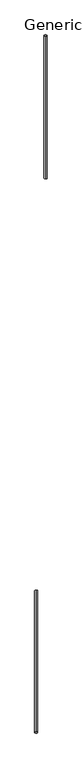
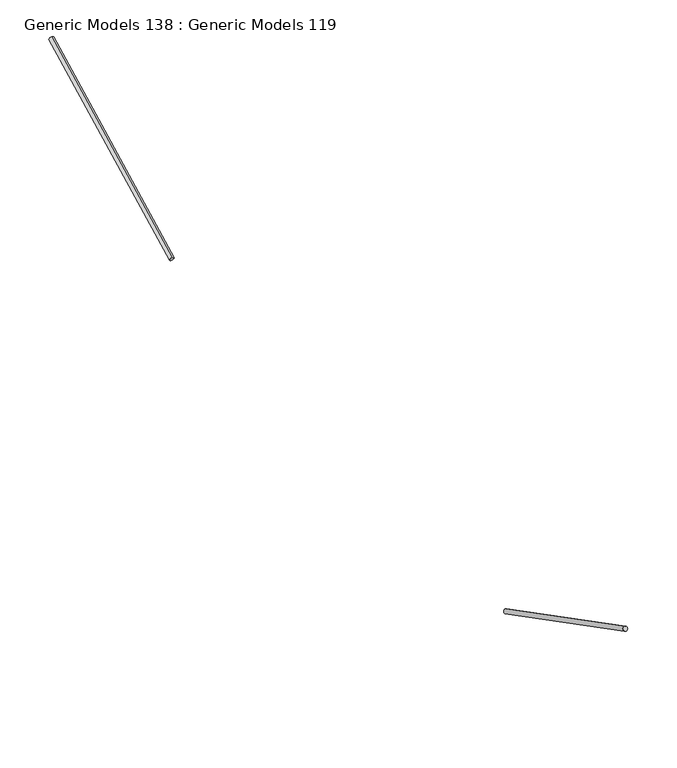
"""IFC4 building model written with IfcOpenShell, lengths in millimetres: proxy geometry, Generic Models 138 : Generic Models 119."""

from ifc_helpers import new_model, si_unit, point, frame, origin, place, context, project, spatial, circle_curve, trimmed, source, transform, mapped, element, save
from ifc_brep_helpers import plane_surface, extruded_surface, advanced_brep


def generic_models_138_generic_models_119_a440c868(model_context):
    return source(origin(), model_context, "Body", "AdvancedBrep", [
        advanced_brep(
        [(32003.9965778, 34299.9490581, 268227.7367968), (32003.9965778, 34308.6764571, 268210.8035453), (32002.4450787, 35180.4781368, 268681.5615446), (32002.4450787, 35189.2055358, 268664.6282931)],
        [
            (0, 1, circle_curve(frame((32003.9965778, 34304.3127576, 268219.270171), z_axis=(0.0, -0.8888845937971532, -0.4581311808969894), x_axis=(0.0, 0.4581311808969894, -0.8888845937971532)), 9.525)),
            (1, 0, circle_curve(frame((32003.9965778, 34304.3127576, 268219.270171), z_axis=(0.0, -0.8888845937971532, -0.4581311808969894), x_axis=(0.0, 0.4581311808969894, -0.8888845937971532)), 9.525)),
            (2, 3, circle_curve(frame((32002.4450787, 35184.8418363, 268673.0949188), z_axis=(0.0, 0.8888845937971532, 0.4581311808969894), x_axis=(0.0, 0.4581311808969894, -0.8888845937971532)), 9.525)),
            (3, 2, circle_curve(frame((32002.4450787, 35184.8418363, 268673.0949188), z_axis=(0.0, 0.8888845937971532, 0.4581311808969894), x_axis=(0.0, 0.4581311808969894, -0.8888845937971532)), 9.525)),
            (3, 1),
            (0, 2),
        ],
        [
            plane_surface(frame((32003.9965778, 34304.3127576, 268219.270171), z_axis=(0.0, -0.8888845937971532, -0.4581311808969894), x_axis=(-1.0, 0.0, 0.0))),
            plane_surface(frame((32002.4450787, 35184.8418363, 268673.0949188), z_axis=(0.0, 0.8888845937971532, 0.4581311808969894), x_axis=(-1.0, 0.0, 0.0))),
            extruded_surface(trimmed(circle_curve(frame((32002.4450787, 35184.8418363, 268673.0949188), z_axis=(0.0, -0.8888845937971532, -0.4581311808969894), x_axis=(0.0, 0.4581311808969894, -0.8888845937971532)), 9.525), [point((32002.4450787, 35180.4781368, 268681.5615446))], [point((32002.4450787, 35189.2055358, 268664.6282931))], True, "CARTESIAN"), (1.55149910000182, -880.5290787000049, -453.8247478000121), 990.6012150716763),
            extruded_surface(trimmed(circle_curve(frame((32002.4450787, 35184.8418363, 268673.0949188), z_axis=(0.0, -0.8888845937971532, -0.4581311808969894), x_axis=(0.0, 0.4581311808969894, -0.8888845937971532)), 9.525), [point((32002.4450787, 35189.2055358, 268664.6282931))], [point((32002.4450787, 35180.4781368, 268681.5615446))], True, "CARTESIAN"), (1.55149910000182, -880.5290787000049, -453.8247478000121), 990.6012150716763),
        ],
        [
            (0, [[1, 2]]),
            (1, [[3, 4]]),
            (2, [[-4, 5, -1, 6]]),
            (3, [[-3, -6, -2, -5]]),
        ],
    ),
        advanced_brep(
        [(31945.3483901, 31748.297289, 268203.9793966), (31945.3483901, 31757.0482414, 268220.9004879), (31945.2937775, 30874.0409026, 268656.1119362), (31945.2937775, 30882.791855, 268673.0330276)],
        [
            (0, 1, circle_curve(frame((31945.3483901, 31752.6727652, 268212.4399422), z_axis=(0.0, 0.8882462650221944, -0.459367579041144), x_axis=(0.0, 0.459367579041144, 0.8882462650221944)), 9.525)),
            (1, 0, circle_curve(frame((31945.3483901, 31752.6727652, 268212.4399422), z_axis=(0.0, 0.8882462650221944, -0.459367579041144), x_axis=(0.0, 0.459367579041144, 0.8882462650221944)), 9.525)),
            (2, 3, circle_curve(frame((31945.2937775, 30878.4163788, 268664.5724819), z_axis=(0.0, -0.8882462650221944, 0.459367579041144), x_axis=(0.0, 0.459367579041144, 0.8882462650221944)), 9.525)),
            (3, 2, circle_curve(frame((31945.2937775, 30878.4163788, 268664.5724819), z_axis=(0.0, -0.8882462650221944, 0.459367579041144), x_axis=(0.0, 0.459367579041144, 0.8882462650221944)), 9.525)),
            (3, 1),
            (0, 2),
        ],
        [
            plane_surface(frame((31945.3483901, 31752.6727652, 268212.4399422), z_axis=(0.0, 0.8882462650221944, -0.459367579041144), x_axis=(-1.0, 0.0, 0.0))),
            plane_surface(frame((31945.2937775, 30878.4163788, 268664.5724819), z_axis=(0.0, -0.8882462650221944, 0.459367579041144), x_axis=(-1.0, 0.0, 0.0))),
            extruded_surface(trimmed(circle_curve(frame((31945.2937775, 30878.4163788, 268664.5724819), z_axis=(0.0, 0.8882462650221944, -0.459367579041144), x_axis=(0.0, 0.459367579041144, 0.8882462650221944)), 9.525), [point((31945.2937775, 30874.0409026, 268656.1119362))], [point((31945.2937775, 30882.791855, 268673.0330276))], True, "CARTESIAN"), (0.05461260000083712, 874.2563864000003, -452.13253969996003), 984.2500015744266),
            extruded_surface(trimmed(circle_curve(frame((31945.2937775, 30878.4163788, 268664.5724819), z_axis=(0.0, 0.8882462650221944, -0.459367579041144), x_axis=(0.0, 0.459367579041144, 0.8882462650221944)), 9.525), [point((31945.2937775, 30882.791855, 268673.0330276))], [point((31945.2937775, 30874.0409026, 268656.1119362))], True, "CARTESIAN"), (0.05461260000083712, 874.2563864000003, -452.13253969996003), 984.2500015744266),
        ],
        [
            (0, [[1, 2]]),
            (1, [[3, 4]]),
            (2, [[-4, 5, -1, 6]]),
            (3, [[-3, -6, -2, -5]]),
        ],
    ),
    ])


if __name__ == "__main__":
    model = new_model("IFC4")
    model_context = context("Model", 3, world=origin())
    ifc_project = project(units=[si_unit("LENGTHUNIT", "METRE", prefix="MILLI")], contexts=[model_context])
    site = spatial("IfcSite", under=ifc_project)
    building = spatial("IfcBuilding", under=site)
    placement = place(None, origin())
    generic_models_138_generic_models_119_shape = generic_models_138_generic_models_119_a440c868(model_context)
    element("IfcBuildingElementProxy", 1, Name="Generic Models 138 : Generic Models 119", ObjectType="Generic Models 138 : Generic Models 119", at=placement, inside=building, context=model_context, shape_type="MappedRepresentation", body=[
        mapped(generic_models_138_generic_models_119_shape, transform((0.0, 0.0, 0.0), x_axis=(1.0, 0.0, 0.0), y_axis=(0.0, 1.0, 0.0), z_axis=(0.0, 0.0, 1.0))),
    ])
    save(model, "model.ifc")

# Revit data of these elements
# Element 1 (IfcBuildingElementProxy, "Generic Models 138 : Generic Models 119")
#   Materials on its faces: "3/4\" DIA. ROD"
# Materials
#   "3/4\" DIA. ROD": class "Metal", colour RGB 199 199 199, transparency 0, Description = "Carbon steel", Cost = 0
